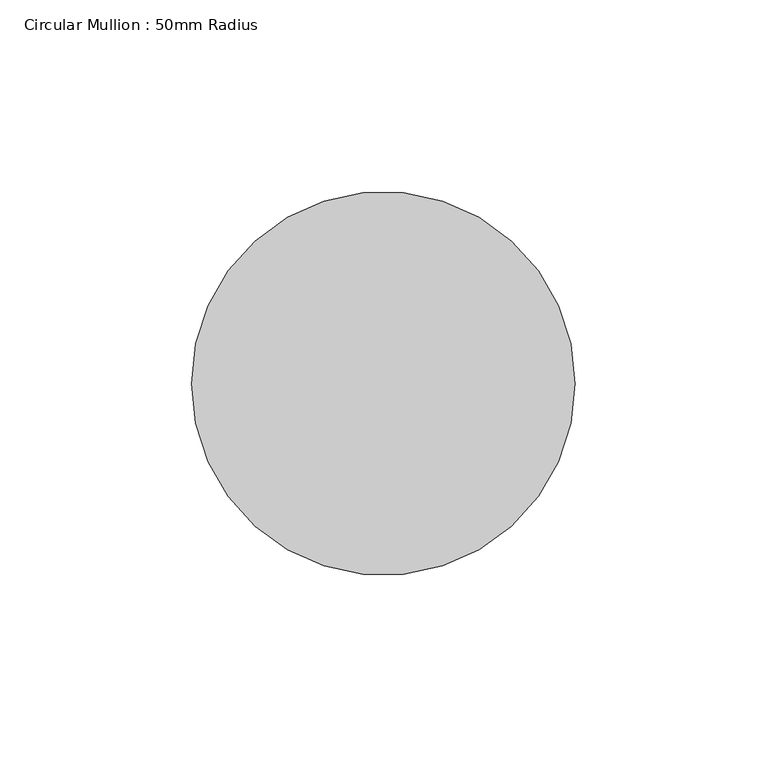
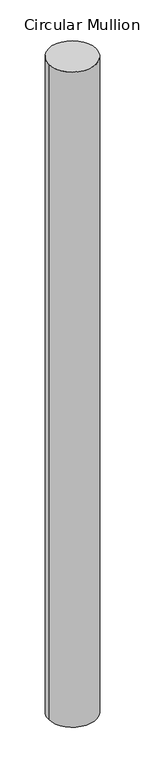
"""IFC4 building model written with IfcOpenShell, lengths in millimetres: member geometry, Circular Mullion : 50mm Radius."""

from ifc_helpers import new_model, si_unit, point, frame, origin, origin_2d, place, context, project, spatial, circle_curve, trimmed, segment, composite_curve, outline, extrude, source, transform, mapped, element, save


def circular_mullion_50mm_radius_e39b39b8(model_context):
    return source(origin(), model_context, "Body", "SweptSolid", [
        extrude(outline(composite_curve([segment(trimmed(circle_curve(origin_2d(), 50.0), [point((50.0, 0.0))], [point((-50.0, 0.0))], False, "CARTESIAN"), True, "CONTINUOUS"), segment(trimmed(circle_curve(origin_2d(), 50.0), [point((-50.0, 0.0))], [point((50.0, 0.0))], False, "CARTESIAN"), True, "CONTINUOUS")], self_intersect=False)), frame((0.0, 0.0, -1458.3812141), z_axis=(0.0, 0.0, 1.0), x_axis=(1.0, 0.0, 0.0)), (0.0, 0.0, 1.0), 1458.3812141),
    ])


if __name__ == "__main__":
    model = new_model("IFC4")
    model_context = context("Model", 3, world=origin())
    ifc_project = project(units=[si_unit("LENGTHUNIT", "METRE", prefix="MILLI")], contexts=[model_context])
    site = spatial("IfcSite", under=ifc_project)
    building = spatial("IfcBuilding", under=site)
    placement = place(None, origin())
    circular_mullion_50mm_radius_shape = circular_mullion_50mm_radius_e39b39b8(model_context)
    element("IfcMember", 1, ObjectType="Circular Mullion : 50mm Radius", at=placement, inside=building, context=model_context, shape_type="MappedRepresentation", body=[
        mapped(circular_mullion_50mm_radius_shape, transform((0.0, 0.0, 0.0), x_axis=(1.0, 0.0, 0.0), y_axis=(0.0, 1.0, 0.0), z_axis=(0.0, 0.0, 1.0))),
    ])
    save(model, "model.ifc")

# Revit data of these elements
# Type "Circular Mullion : 50mm Radius"
#   built-in parameter 1007350 = 0.164042 (stored number, unit not read)
# Element 1 (IfcMember, "Circular Mullion : 50mm Radius")
#   Materials on its faces: "Aluminium"
# Materials
#   "Aluminium": class "Metal", colour RGB 247 247 247, transparency 0, Description = "Aluminium 6061", Cost = 0
